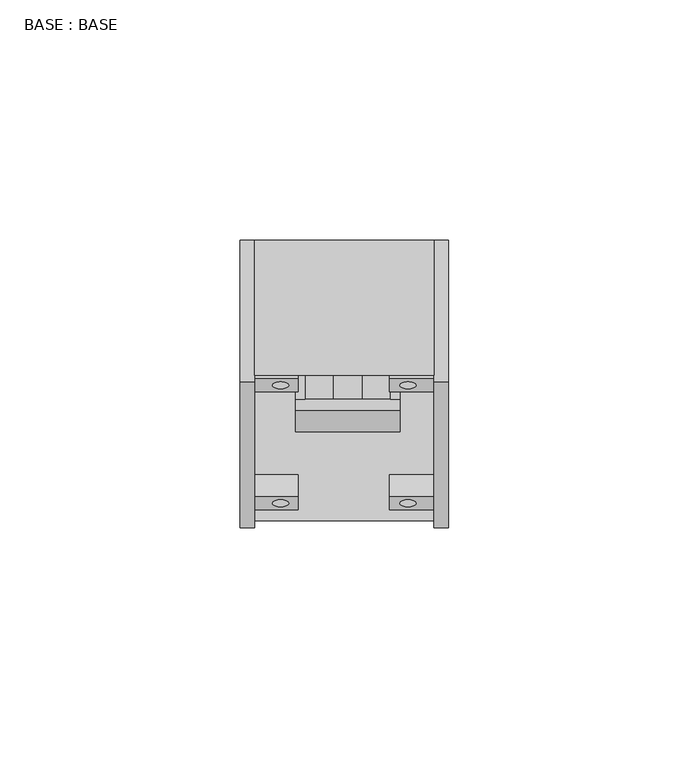
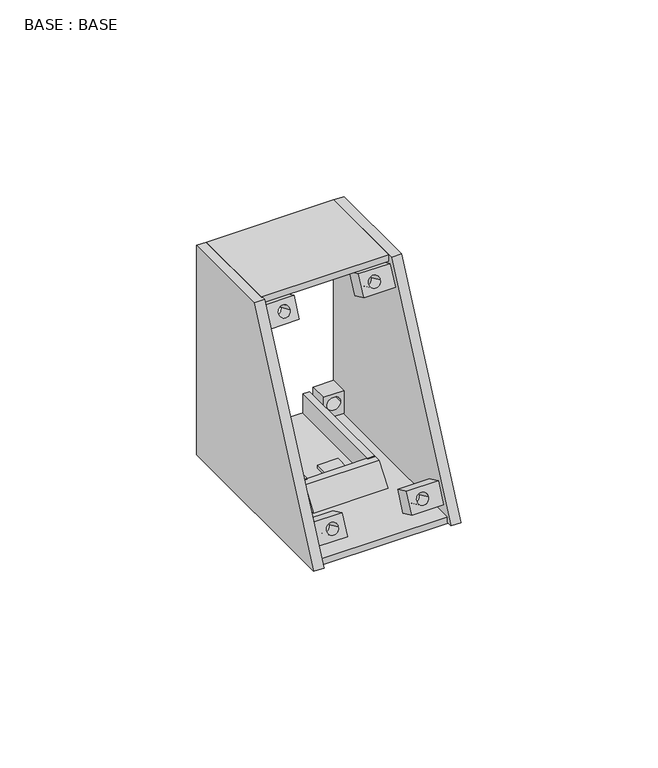
"""IFC4 building model written with IfcOpenShell, lengths in millimetres: proxy geometry, BASE : BASE."""

from ifc_helpers import new_model, si_unit, point, frame, frame_2d, origin, origin_with_axes, place, context, project, spatial, polyline, circle_curve, trimmed, segment, composite_curve, outline, extrude, source, transform, mapped, element, save


def base_base_a5933ecb(model_context):
    return source(origin(), model_context, "Body", "SweptSolid", [
        extrude(outline(polyline([(3.2, -2.2), (-3.2, -2.2), (-3.2, 7.1), (3.2, 7.1), (3.2, -2.2)]), holes=[composite_curve([segment(trimmed(circle_curve(frame_2d((0.0, 1.7)), 1.7), [point((0.0, 0.0))], [point((0.0, 3.4))], True, "CARTESIAN"), True, "CONTINUOUS"), segment(trimmed(circle_curve(frame_2d((0.0, 1.7)), 1.7), [point((0.0, 3.4))], [point((0.0, 0.0))], True, "CARTESIAN"), True, "CONTINUOUS")], self_intersect=False)]), frame((2402.2719295, 1326.1385366, 57.7208133), z_axis=(0.0, -0.9063077870366535, 0.4226182617406919), x_axis=(0.0, -0.4226182617406919, -0.9063077870366535)), (0.0, 0.0, 1.0), 5.0),
        extrude(outline(polyline([(3.2, -30.2), (-3.2, -30.2), (-3.2, -21.2), (3.2, -21.2), (3.2, -30.2)]), holes=[composite_curve([segment(trimmed(circle_curve(frame_2d((0.0, -24.8)), 1.7), [point((0.0, -23.1))], [point((0.0, -26.5))], True, "CARTESIAN"), True, "CONTINUOUS"), segment(trimmed(circle_curve(frame_2d((0.0, -24.8)), 1.7), [point((0.0, -26.5))], [point((0.0, -23.1))], True, "CARTESIAN"), True, "CONTINUOUS")], self_intersect=False)]), frame((2402.2719295, 1326.1385366, 57.7208133), z_axis=(0.0, -0.9063077870366535, 0.4226182617406919), x_axis=(0.0, -0.4226182617406919, -0.9063077870366535)), (0.0, 0.0, 1.0), 5.0),
        extrude(outline(polyline([(61.2, -2.2), (54.8, -2.2), (54.8, 7.1), (61.2, 7.1), (61.2, -2.2)]), holes=[composite_curve([segment(trimmed(circle_curve(frame_2d((58.0000001, 1.7)), 1.7), [point((58.0000001, 3.4))], [point((58.0000001, 0.0))], True, "CARTESIAN"), True, "CONTINUOUS"), segment(trimmed(circle_curve(frame_2d((58.0000001, 1.7)), 1.7), [point((58.0000001, 0.0))], [point((58.0000001, 3.4))], True, "CARTESIAN"), True, "CONTINUOUS")], self_intersect=False)]), frame((2402.2719295, 1326.1385366, 57.7208133), z_axis=(0.0, -0.9063077870366535, 0.4226182617406919), x_axis=(0.0, -0.4226182617406919, -0.9063077870366535)), (0.0, 0.0, 1.0), 5.0),
        extrude(outline(polyline([(61.2, -21.2), (61.2, -30.2), (54.8, -30.2), (54.8, -21.2), (61.2, -21.2)]), holes=[composite_curve([segment(trimmed(circle_curve(frame_2d((58.0000001, -24.8)), 1.7), [point((58.0000001, -23.1))], [point((58.0000001, -26.5))], True, "CARTESIAN"), True, "CONTINUOUS"), segment(trimmed(circle_curve(frame_2d((58.0000001, -24.8)), 1.7), [point((58.0000001, -26.5))], [point((58.0000001, -23.1))], True, "CARTESIAN"), True, "CONTINUOUS")], self_intersect=False)]), frame((2402.2719295, 1326.1385366, 57.7208133), z_axis=(0.0, -0.9063077870366535, 0.4226182617406919), x_axis=(0.0, -0.4226182617406919, -0.9063077870366535)), (0.0, 0.0, 1.0), 5.0),
        extrude(outline(polyline([(2394.4431854, 1318.7384159), (2388.4431854, 1318.7384159), (2388.4431854, 1323.7384159), (2394.4431854, 1323.7384159), (2394.4431854, 1318.7384159)])), frame((0.0, 0.0, 6.0), z_axis=(0.0, 0.0, 1.0), x_axis=(1.0, 0.0, 0.0)), (0.0, 0.0, 1.0), 1.0),
        extrude(outline(polyline([(1336.0781618, 2.0), (1344.7384159, 17.0), (1351.7384159, 17.0), (1351.7384159, 15.25), (1346.4884159, 15.25), (1346.4884159, 2.0), (1336.0781618, 2.0)])), frame((2372.0719295, 0.0, 0.0), z_axis=(1.0, 0.0, 0.0), x_axis=(0.0, 1.0, 0.0)), (0.0, 0.0, 1.0), 6.0),
        extrude(outline(polyline([(2409.3719295, 1323.7384159), (2372.0719295, 1323.7384159), (2372.0719295, 1351.7384159), (2409.3719295, 1351.7384159), (2409.3719295, 1323.7384159)])), frame((0.0, 0.0, 63.0), z_axis=(0.0, 0.0, 1.0), x_axis=(1.0, 0.0, 0.0)), (0.0, 0.0, 1.0), 2.0),
        extrude(outline(polyline([(2.0, 2403.3719295), (2.0, 2409.3719295), (9.0, 2409.3719295), (9.0, 2403.3719295), (2.0, 2403.3719295)]), holes=[composite_curve([segment(trimmed(circle_curve(frame_2d((6.0, 2406.3719295)), 2.0), [point((6.0, 2408.3719295))], [point((6.0, 2404.3719295))], True, "CARTESIAN"), True, "CONTINUOUS"), segment(trimmed(circle_curve(frame_2d((6.0, 2406.3719295)), 2.0), [point((6.0, 2404.3719295))], [point((6.0, 2408.3719295))], True, "CARTESIAN"), True, "CONTINUOUS")], self_intersect=False)]), frame((0.0, 1346.4884159, 0.0), z_axis=(0.0, 1.0, 0.0), x_axis=(0.0, 0.0, 1.0)), (0.0, 0.0, 1.0), 5.25),
        extrude(outline(polyline([(2.0, 2378.0719295), (9.0, 2378.0719295), (9.0, 2372.0719295), (2.0, 2372.0719295), (2.0, 2378.0719295)]), holes=[composite_curve([segment(trimmed(circle_curve(frame_2d((6.0, 2375.0719295)), 2.0), [point((6.0, 2377.0719295))], [point((6.0, 2373.0719295))], True, "CARTESIAN"), True, "CONTINUOUS"), segment(trimmed(circle_curve(frame_2d((6.0, 2375.0719295)), 2.0), [point((6.0, 2373.0719295))], [point((6.0, 2377.0719295))], True, "CARTESIAN"), True, "CONTINUOUS")], self_intersect=False)]), frame((0.0, 1346.4884159, 0.0), z_axis=(0.0, 1.0, 0.0), x_axis=(0.0, 0.0, 1.0)), (0.0, 0.0, 1.0), 5.25),
        extrude(outline(polyline([(63.0, 2403.3719295), (56.0, 2403.3719295), (56.0, 2409.3719295), (63.0, 2409.3719295), (63.0, 2403.3719295)]), holes=[composite_curve([segment(trimmed(circle_curve(frame_2d((59.0, 2406.3719295)), 2.0), [point((59.0, 2408.3719295))], [point((59.0, 2404.3719295))], True, "CARTESIAN"), True, "CONTINUOUS"), segment(trimmed(circle_curve(frame_2d((59.0, 2406.3719295)), 2.0), [point((59.0, 2404.3719295))], [point((59.0, 2408.3719295))], True, "CARTESIAN"), True, "CONTINUOUS")], self_intersect=False)]), frame((0.0, 1346.4884159, 0.0), z_axis=(0.0, 1.0, 0.0), x_axis=(0.0, 0.0, 1.0)), (0.0, 0.0, 1.0), 5.25),
        extrude(outline(polyline([(63.0, 2378.0719295), (63.0, 2372.0719295), (56.0, 2372.0719295), (56.0, 2378.0719295), (63.0, 2378.0719295)]), holes=[composite_curve([segment(trimmed(circle_curve(frame_2d((59.0, 2375.0719295)), 2.0), [point((59.0, 2377.0719295))], [point((59.0, 2373.0719295))], True, "CARTESIAN"), True, "CONTINUOUS"), segment(trimmed(circle_curve(frame_2d((59.0, 2375.0719295)), 2.0), [point((59.0, 2373.0719295))], [point((59.0, 2377.0719295))], True, "CARTESIAN"), True, "CONTINUOUS")], self_intersect=False)]), frame((0.0, 1346.4884159, 0.0), z_axis=(0.0, 1.0, 0.0), x_axis=(0.0, 0.0, 1.0)), (0.0, 0.0, 1.0), 5.25),
        extrude(outline(polyline([(1351.7384159, 0.0), (1292.0509228, 0.0), (1322.3609206, 65.0), (1351.7384159, 65.0), (1351.7384159, 0.0)])), frame((2409.3719295, 0.0, 0.0), z_axis=(1.0, 0.0, 0.0), x_axis=(0.0, 1.0, 0.0)), (0.0, 0.0, 1.0), 3.0),
        extrude(outline(polyline([(1351.7384159, 0.0), (1292.0509228, 0.0), (1322.3609206, 65.0), (1351.7384159, 65.0), (1351.7384159, 0.0)])), frame((2369.0719295, 0.0, 0.0), z_axis=(1.0, 0.0, 0.0), x_axis=(0.0, 1.0, 0.0)), (0.0, 0.0, 1.0), 3.0),
        extrude(outline(polyline([(2402.3331854, 1318.7384159), (2400.3331854, 1318.7384159), (2400.3331854, 1351.7384159), (2402.3331854, 1351.7384159), (2402.3331854, 1318.7384159)])), frame((0.0, 0.0, 2.0), z_axis=(0.0, 0.0, 1.0), x_axis=(1.0, 0.0, 0.0)), (0.0, 0.0, 1.0), 6.0),
        extrude(outline(polyline([(2380.5531854, 1318.7384159), (2380.5531854, 1351.7384159), (2382.5531854, 1351.7384159), (2382.5531854, 1318.7384159), (2380.5531854, 1318.7384159)])), frame((0.0, 0.0, 2.0), z_axis=(0.0, 0.0, 1.0), x_axis=(1.0, 0.0, 0.0)), (0.0, 0.0, 1.0), 6.0),
        extrude(outline(polyline([(1318.7384159, 8.0), (1318.7384159, 2.0), (1311.9905964, 2.0), (1316.4775131, 8.0), (1318.7384159, 8.0)])), frame((2380.5531854, 0.0, 0.0), z_axis=(1.0, 0.0, 0.0), x_axis=(0.0, 1.0, 0.0)), (0.0, 0.0, 1.0), 21.78),
        extrude(outline(polyline([(2409.3719295, 1293.4498458), (2372.0719295, 1293.4498458), (2372.0719295, 1351.7384159), (2409.3719295, 1351.7384159), (2409.3719295, 1293.4498458)])), origin_with_axes(), (0.0, 0.0, 1.0), 2.0),
    ])


if __name__ == "__main__":
    model = new_model("IFC4")
    model_context = context("Model", 3, world=origin())
    ifc_project = project(units=[si_unit("LENGTHUNIT", "METRE", prefix="MILLI")], contexts=[model_context])
    site = spatial("IfcSite", under=ifc_project)
    building = spatial("IfcBuilding", under=site)
    placement = place(None, origin())
    base_base_shape = base_base_a5933ecb(model_context)
    element("IfcBuildingElementProxy", 1, Name="BASE : BASE", ObjectType="BASE : BASE", at=placement, inside=building, context=model_context, shape_type="MappedRepresentation", body=[
        mapped(base_base_shape, transform((0.0, 0.0, 0.0), x_axis=(1.0, 0.0, 0.0), y_axis=(0.0, 1.0, 0.0), z_axis=(0.0, 0.0, 1.0))),
    ])
    save(model, "model.ifc")

# Revit data of these elements
# Element 1 (IfcBuildingElementProxy, "BASE : BASE")
#   Materials on its faces: ".BOX LATERAL"
# Materials
#   ".BOX LATERAL": class "Vidro", colour RGB 236 240 239, transparency 0.15, Cost = 0
